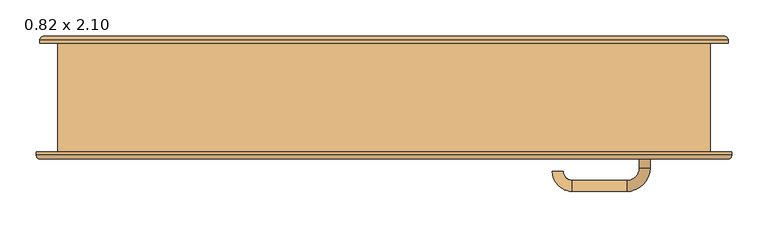
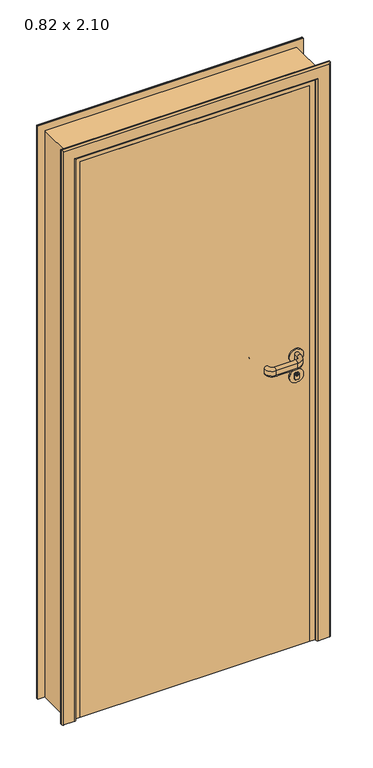
"""IFC4 building model written with IfcOpenShell, lengths in millimetres: door geometry, CC_PORTA ABRIR_1 FOLHA LISA : 0.82 x 2.10."""

from ifc_helpers import new_model, si_unit, point, frame, frame_2d, origin, origin_with_axes, place, context, project, spatial, polyline, circle_curve, ellipse_curve, trimmed, segment, composite_curve, outline, extrude, faceted_brep, source, transform, mapped, element, save
from ifc_brep_helpers import plane_surface, cylinder_surface, revolved_surface, advanced_brep


def door_0_82_x_2_10_6c23dadb(model_context):
    return source(origin(), model_context, "Body", "SolidModel", [
        advanced_brep(
        [(352.5, -40.0, 1091.5062746), (367.5, -40.0, 1091.5062746), (367.5, -40.0, 1108.3826844), (352.5, -40.0, 1108.3826844), (367.5, -18.0, 1091.5062746), (367.5, -18.0, 1108.3826844), (352.5, -18.0, 1108.3826844), (352.5, -18.0, 1091.5062746), (335.0, 14.5, 1108.3826844), (335.0, 14.5, 1091.5062746), (260.0, 14.5, 1091.5062746), (260.0, 14.5, 1108.3826844), (335.0, -0.5, 1091.5062746), (335.0, -0.5, 1108.3826844), (260.0, -0.5, 1108.3826844), (260.0, -0.5, 1091.5062746), (247.5, -13.0, 1091.5062746), (247.5, -13.0, 1108.3826844), (232.5, -13.0, 1108.3826844), (232.5, -13.0, 1091.5062746)],
        [
            (0, 1, circle_curve(frame((360.0, -40.0, 1091.5062746), z_axis=(0.0, -1.0, 0.0), x_axis=(0.0, 0.0, 1.0)), 7.5)),
            (1, 2),
            (2, 3, circle_curve(frame((360.0, -40.0, 1108.3826844), z_axis=(0.0, -1.0, 0.0), x_axis=(0.0, 0.0, 1.0)), 7.5)),
            (3, 0),
            (1, 4),
            (4, 5),
            (5, 2),
            (3, 6),
            (6, 7),
            (7, 0),
            (8, 9),
            (9, 10),
            (10, 11),
            (11, 8),
            (12, 13),
            (13, 14),
            (14, 15),
            (15, 12),
            (7, 4, circle_curve(frame((360.0, -18.0, 1091.5062746), z_axis=(0.0, -1.0, 0.0), x_axis=(0.0, 0.0, 1.0)), 7.5)),
            (5, 6, circle_curve(frame((360.0, -18.0, 1108.3826844), z_axis=(0.0, -1.0, 0.0), x_axis=(0.0, 0.0, 1.0)), 7.5)),
            (9, 12, circle_curve(frame((335.0, 7.0, 1091.5062746), z_axis=(-1.0, 0.0, 0.0), x_axis=(0.0, 0.0, 1.0)), 7.5)),
            (15, 10, circle_curve(frame((260.0, 7.0, 1091.5062746), z_axis=(1.0, 0.0, 0.0), x_axis=(0.0, 0.0, 1.0)), 7.5)),
            (13, 8, circle_curve(frame((335.0, 7.0, 1108.3826844), z_axis=(-1.0, 0.0, 0.0), x_axis=(0.0, 0.0, 1.0)), 7.5)),
            (11, 14, circle_curve(frame((260.0, 7.0, 1108.3826844), z_axis=(1.0, 0.0, 0.0), x_axis=(0.0, 0.0, 1.0)), 7.5)),
            (9, 4, circle_curve(frame((335.0, -18.0, 1091.5062746), z_axis=(0.0, 0.0, -1.0), x_axis=(1.0, 0.0, 0.0)), 32.5)),
            (7, 12, circle_curve(frame((335.0, -18.0, 1091.5062746), z_axis=(0.0, 0.0, 1.0), x_axis=(1.0, 0.0, 0.0)), 17.5)),
            (8, 5, circle_curve(frame((335.0, -18.0, 1108.3826844), z_axis=(0.0, 0.0, -1.0), x_axis=(1.0, 0.0, 0.0)), 32.5)),
            (13, 6, circle_curve(frame((335.0, -18.0, 1108.3826844), z_axis=(0.0, 0.0, -1.0), x_axis=(1.0, 0.0, 0.0)), 17.5)),
            (16, 17),
            (17, 18, circle_curve(frame((240.0, -13.0, 1108.3826844), z_axis=(0.0, -1.0, 0.0), x_axis=(0.0, 0.0, 1.0)), 7.5)),
            (18, 19),
            (19, 16, circle_curve(frame((240.0, -13.0, 1091.5062746), z_axis=(0.0, -1.0, 0.0), x_axis=(0.0, 0.0, 1.0)), 7.5)),
            (19, 10, circle_curve(frame((260.0, -13.0, 1091.5062746), z_axis=(0.0, 0.0, -1.0), x_axis=(0.0, 1.0, 0.0)), 27.5)),
            (15, 16, circle_curve(frame((260.0, -13.0, 1091.5062746), z_axis=(0.0, 0.0, 1.0), x_axis=(0.0, 1.0, 0.0)), 12.5)),
            (18, 11, circle_curve(frame((260.0, -13.0, 1108.3826844), z_axis=(0.0, 0.0, -1.0), x_axis=(0.0, 1.0, 0.0)), 27.5)),
            (17, 14, circle_curve(frame((260.0, -13.0, 1108.3826844), z_axis=(0.0, 0.0, -1.0), x_axis=(0.0, 1.0, 0.0)), 12.5)),
        ],
        [
            plane_surface(frame((360.0, -40.0, 1099.9444795), z_axis=(0.0, -1.0, 0.0), x_axis=(0.0, 0.0, 1.0))),
            plane_surface(frame((367.5, -40.0, 1091.5062746), z_axis=(1.0, 0.0, 0.0), x_axis=(0.0, 1.0, 0.0))),
            plane_surface(frame((352.5, -40.0, 1108.3826844), z_axis=(-1.0, 0.0, 0.0), x_axis=(0.0, 1.0, 0.0))),
            plane_surface(frame((335.0, 14.5, 1091.5062746), z_axis=(0.0, 1.0, 0.0), x_axis=(-1.0, 0.0, 0.0))),
            plane_surface(frame((335.0, -0.5, 1108.3826844), z_axis=(0.0, -1.0, 0.0), x_axis=(-1.0, 0.0, 0.0))),
            cylinder_surface(frame((360.0, -40.0, 1091.5062746), z_axis=(0.0, -1.0, 0.0), x_axis=(0.0, 0.0, 1.0)), 7.5),
            cylinder_surface(frame((360.0, -40.0, 1108.3826844), z_axis=(0.0, -1.0, 0.0), x_axis=(0.0, 0.0, 1.0)), 7.5),
            cylinder_surface(frame((335.0, 7.0, 1091.5062746), z_axis=(1.0, 0.0, 0.0), x_axis=(0.0, 0.0, 1.0)), 7.5),
            cylinder_surface(frame((335.0, 7.0, 1108.3826844), z_axis=(1.0, 0.0, 0.0), x_axis=(0.0, 0.0, 1.0)), 7.5),
            revolved_surface(trimmed(ellipse_curve(frame((360.0, -18.0, 1091.5062746), z_axis=(0.0, -1.0, 0.0), x_axis=(0.0, 0.0, 1.0)), 7.5, 7.5), [point((352.5, -18.0, 1091.5062746))], [point((367.5, -18.0, 1091.5062746))], True, "CARTESIAN"), (335.0, -18.0, 1099.9444795), (0.0, 0.0, 1.0)),
            cylinder_surface(frame((335.0, -18.0, 1099.9444795), z_axis=(0.0, 0.0, 1.0), x_axis=(1.0, 0.0, 0.0)), 32.5),
            revolved_surface(trimmed(ellipse_curve(frame((360.0, -18.0, 1108.3826844), z_axis=(0.0, -1.0, 0.0), x_axis=(0.0, 0.0, 1.0)), 7.5, 7.5), [point((367.5, -18.0, 1108.3826844))], [point((352.5, -18.0, 1108.3826844))], True, "CARTESIAN"), (335.0, -18.0, 1099.9444795), (0.0, 0.0, 1.0)),
            revolved_surface(polyline([(352.5, -18.0, 1108.3826844), (352.5, -18.0, 1091.5062746)]), (335.0, -18.0, 1099.9444795), (0.0, 0.0, 1.0)),
            plane_surface(frame((240.0, -13.0, 1099.9444795), z_axis=(0.0, -1.0, 0.0), x_axis=(0.0, 0.0, 1.0))),
            revolved_surface(trimmed(ellipse_curve(frame((260.0, 7.0, 1091.5062746), z_axis=(1.0, 0.0, 0.0), x_axis=(0.0, 0.0, 1.0)), 7.5, 7.5), [point((260.0, -0.5, 1091.5062746))], [point((260.0, 14.5, 1091.5062746))], True, "CARTESIAN"), (260.0, -13.0, 1099.9444795), (0.0, 0.0, 1.0)),
            cylinder_surface(frame((260.0, -13.0, 1099.9444795), z_axis=(0.0, 0.0, 1.0), x_axis=(0.0, 1.0, 0.0)), 27.5),
            revolved_surface(trimmed(ellipse_curve(frame((260.0, 7.0, 1108.3826844), z_axis=(1.0, 0.0, 0.0), x_axis=(0.0, 0.0, 1.0)), 7.5, 7.5), [point((260.0, 14.5, 1108.3826844))], [point((260.0, -0.5, 1108.3826844))], True, "CARTESIAN"), (260.0, -13.0, 1099.9444795), (0.0, 0.0, 1.0)),
            revolved_surface(polyline([(260.0, -0.5, 1108.3826844), (260.0, -0.5, 1091.5062746)]), (260.0, -13.0, 1099.9444795), (0.0, 0.0, 1.0)),
        ],
        [
            (0, [[1, 2, 3, 4]]),
            (1, [[-2, 5, 6, 7]]),
            (2, [[-4, 8, 9, 10]]),
            (3, [[11, 12, 13, 14]]),
            (4, [[15, 16, 17, 18]]),
            (5, [[-1, -10, 19, -5]]),
            (6, [[-3, -7, 20, -8]]),
            (7, [[21, -18, 22, -12]]),
            (8, [[23, -14, 24, -16]]),
            (9, [[25, -19, 26, -21]]),
            (10, [[27, -6, -25, -11]]),
            (11, [[28, -20, -27, -23]]),
            (12, [[-26, -9, -28, -15]]),
            (13, [[29, 30, 31, 32]]),
            (14, [[33, -22, 34, -32]]),
            (15, [[35, -13, -33, -31]]),
            (16, [[36, -24, -35, -30]]),
            (17, [[-34, -17, -36, -29]]),
        ],
    ),
        extrude(outline(polyline([(361.0, -40.0), (359.0, -40.0), (359.0, -30.9), (361.0, -30.9), (361.0, -40.0)])), frame((0.0, 0.0, 1027.9555433), z_axis=(0.0, 0.0, 1.0), x_axis=(1.0, 0.0, 0.0)), (0.0, 0.0, 1.0), 7.8071257),
        extrude(outline(composite_curve([segment(trimmed(circle_curve(frame_2d((1031.5611613, 360.0)), 5.0), [point((1036.5611613, 360.0))], [point((1026.5611613, 360.0))], False, "CARTESIAN"), True, "CONTINUOUS"), segment(trimmed(circle_curve(frame_2d((1031.5611613, 360.0)), 5.0), [point((1026.5611613, 360.0))], [point((1036.5611613, 360.0))], False, "CARTESIAN"), True, "CONTINUOUS")], self_intersect=False), holes=[polyline([(1035.7626689, 361.0), (1027.9555433, 361.0), (1027.9555433, 359.0), (1035.7626689, 359.0), (1035.7626689, 361.0)])]), frame((0.0, -40.0, 0.0), z_axis=(0.0, 1.0, 0.0), x_axis=(0.0, 0.0, 1.0)), (0.0, 0.0, 1.0), 10.0),
        extrude(outline(composite_curve([segment(polyline([(1033.4817325, 352.5), (1016.4817325, 352.5)]), True, "CONTINUOUS"), segment(trimmed(circle_curve(frame_2d((1016.4817325, 356.5)), 4.0), [point((1016.4817325, 352.5))], [point((1012.4817325, 356.5))], False, "CARTESIAN"), True, "CONTINUOUS"), segment(polyline([(1012.4817325, 356.5), (1012.4817325, 363.5)]), True, "CONTINUOUS"), segment(trimmed(circle_curve(frame_2d((1016.4817325, 363.5)), 4.0), [point((1012.4817325, 363.5))], [point((1016.4817325, 367.5))], False, "CARTESIAN"), True, "CONTINUOUS"), segment(polyline([(1016.4817325, 367.5), (1033.4817325, 367.5)]), True, "CONTINUOUS"), segment(trimmed(circle_curve(frame_2d((1033.4817325, 363.5)), 4.0), [point((1033.4817325, 367.5))], [point((1037.4817325, 363.5))], False, "CARTESIAN"), True, "CONTINUOUS"), segment(polyline([(1037.4817325, 363.5), (1037.4817325, 356.5)]), True, "CONTINUOUS"), segment(trimmed(circle_curve(frame_2d((1033.4817325, 356.5)), 4.0), [point((1037.4817325, 356.5))], [point((1033.4817325, 352.5))], False, "CARTESIAN"), True, "CONTINUOUS")], self_intersect=False)), frame((0.0, -40.0, 0.0), z_axis=(0.0, 1.0, 0.0), x_axis=(0.0, 0.0, 1.0)), (0.0, 0.0, 1.0), 9.0),
        extrude(outline(composite_curve([segment(trimmed(circle_curve(frame_2d((1099.9444795, 360.0)), 25.0), [point((1124.9444795, 360.0))], [point((1074.9444795, 360.0))], False, "CARTESIAN"), True, "CONTINUOUS"), segment(trimmed(circle_curve(frame_2d((1099.9444795, 360.0)), 25.0), [point((1074.9444795, 360.0))], [point((1124.9444795, 360.0))], False, "CARTESIAN"), True, "CONTINUOUS")], self_intersect=False)), frame((0.0, -40.0, 0.0), z_axis=(0.0, 1.0, 0.0), x_axis=(0.0, 0.0, 1.0)), (0.0, 0.0, 1.0), 6.0),
        extrude(outline(composite_curve([segment(trimmed(circle_curve(frame_2d((1024.9444795, 360.0)), 25.0), [point((1049.9444795, 360.0))], [point((999.9444795, 360.0))], False, "CARTESIAN"), True, "CONTINUOUS"), segment(trimmed(circle_curve(frame_2d((1024.9444795, 360.0)), 25.0), [point((999.9444795, 360.0))], [point((1049.9444795, 360.0))], False, "CARTESIAN"), True, "CONTINUOUS")], self_intersect=False), holes=[composite_curve([segment(trimmed(circle_curve(frame_2d((1033.4817325, 363.5)), 4.0), [point((1037.4817325, 363.5))], [point((1033.4817325, 367.5))], True, "CARTESIAN"), True, "CONTINUOUS"), segment(polyline([(1033.4817325, 367.5), (1016.4817325, 367.5)]), True, "CONTINUOUS"), segment(trimmed(circle_curve(frame_2d((1016.4817325, 363.5)), 4.0), [point((1016.4817325, 367.5))], [point((1012.4817325, 363.5))], True, "CARTESIAN"), True, "CONTINUOUS"), segment(polyline([(1012.4817325, 363.5), (1012.4817325, 356.5)]), True, "CONTINUOUS"), segment(trimmed(circle_curve(frame_2d((1016.4817325, 356.5)), 4.0), [point((1012.4817325, 356.5))], [point((1016.4817325, 352.5))], True, "CARTESIAN"), True, "CONTINUOUS"), segment(polyline([(1016.4817325, 352.5), (1033.4817325, 352.5)]), True, "CONTINUOUS"), segment(trimmed(circle_curve(frame_2d((1033.4817325, 356.5)), 4.0), [point((1033.4817325, 352.5))], [point((1037.4817325, 356.5))], True, "CARTESIAN"), True, "CONTINUOUS"), segment(polyline([(1037.4817325, 356.5), (1037.4817325, 363.5)]), True, "CONTINUOUS")], self_intersect=False)]), frame((0.0, -40.0, 0.0), z_axis=(0.0, 1.0, 0.0), x_axis=(0.0, 0.0, 1.0)), (0.0, 0.0, 1.0), 6.0),
        extrude(outline(polyline([(361.0, -84.1), (359.0, -84.1), (359.0, -75.0), (361.0, -75.0), (361.0, -84.1)])), frame((0.0, 0.0, 1027.9555433), z_axis=(0.0, 0.0, 1.0), x_axis=(1.0, 0.0, 0.0)), (0.0, 0.0, 1.0), 7.8071257),
        advanced_brep(
        [(360.0, -85.0, 1036.5611613), (360.0, -85.0, 1026.5611613), (361.0, -85.0, 1035.7626689), (361.0, -85.0, 1027.9555433), (359.0, -85.0, 1027.9555433), (359.0, -85.0, 1035.7626689), (360.0, -75.0, 1049.9444795), (360.0, -75.0, 999.9444795), (360.0, -84.0, 1036.5611613), (360.0, -84.0, 1026.5611613), (361.0, -84.0, 1035.7626689), (361.0, -84.0, 1027.9555433), (359.0, -84.0, 1027.9555433), (359.0, -84.0, 1035.7626689), (352.5, -84.0, 1033.4817325), (352.5, -84.0, 1016.4817325), (356.5, -84.0, 1012.4817325), (363.5, -84.0, 1012.4817325), (367.5, -84.0, 1016.4817325), (367.5, -84.0, 1033.4817325), (363.5, -84.0, 1037.4817325), (356.5, -84.0, 1037.4817325), (352.5, -81.0, 1033.4817325), (352.5, -81.0, 1016.4817325), (356.5, -81.0, 1012.4817325), (363.5, -81.0, 1012.4817325), (367.5, -81.0, 1016.4817325), (367.5, -81.0, 1033.4817325), (363.5, -81.0, 1037.4817325), (356.5, -81.0, 1037.4817325), (360.0, -81.0, 1049.9444795), (360.0, -81.0, 999.9444795)],
        [
            (0, 1, circle_curve(frame((360.0, -85.0, 1031.5611613), z_axis=(0.0, -1.0, 0.0), x_axis=(0.0, 0.0, -1.0)), 5.0)),
            (1, 0, circle_curve(frame((360.0, -85.0, 1031.5611613), z_axis=(0.0, -1.0, 0.0), x_axis=(0.0, 0.0, -1.0)), 5.0)),
            (2, 3),
            (3, 4),
            (4, 5),
            (5, 2),
            (6, 7, circle_curve(frame((360.0, -75.0, 1024.9444795), z_axis=(0.0, 1.0, 0.0), x_axis=(0.0, 0.0, -1.0)), 25.0)),
            (7, 6, circle_curve(frame((360.0, -75.0, 1024.9444795), z_axis=(0.0, 1.0, 0.0), x_axis=(0.0, 0.0, -1.0)), 25.0)),
            (0, 8),
            (8, 9, circle_curve(frame((360.0, -84.0, 1031.5611613), z_axis=(0.0, -1.0, 0.0), x_axis=(0.0, 0.0, -1.0)), 5.0)),
            (9, 1),
            (9, 8, circle_curve(frame((360.0, -84.0, 1031.5611613), z_axis=(0.0, -1.0, 0.0), x_axis=(0.0, 0.0, -1.0)), 5.0)),
            (2, 10),
            (10, 11),
            (11, 3),
            (11, 12),
            (12, 4),
            (12, 13),
            (13, 5),
            (13, 10),
            (14, 15),
            (15, 16, circle_curve(frame((356.5, -84.0, 1016.4817325), z_axis=(0.0, -1.0, 0.0), x_axis=(0.0, 0.0, -1.0)), 4.0)),
            (16, 17),
            (17, 18, circle_curve(frame((363.5, -84.0, 1016.4817325), z_axis=(0.0, -1.0, 0.0), x_axis=(0.0, 0.0, -1.0)), 4.0)),
            (18, 19),
            (19, 20, circle_curve(frame((363.5, -84.0, 1033.4817325), z_axis=(0.0, -1.0, 0.0), x_axis=(0.0, 0.0, -1.0)), 4.0)),
            (20, 21),
            (21, 14, circle_curve(frame((356.5, -84.0, 1033.4817325), z_axis=(0.0, -1.0, 0.0), x_axis=(0.0, 0.0, -1.0)), 4.0)),
            (14, 22),
            (22, 23),
            (23, 15),
            (23, 24, circle_curve(frame((356.5, -81.0, 1016.4817325), z_axis=(0.0, -1.0, 0.0), x_axis=(0.0, 0.0, -1.0)), 4.0)),
            (24, 16),
            (24, 25),
            (25, 17),
            (25, 26, circle_curve(frame((363.5, -81.0, 1016.4817325), z_axis=(0.0, -1.0, 0.0), x_axis=(0.0, 0.0, -1.0)), 4.0)),
            (26, 18),
            (26, 27),
            (27, 19),
            (27, 28, circle_curve(frame((363.5, -81.0, 1033.4817325), z_axis=(0.0, -1.0, 0.0), x_axis=(0.0, 0.0, -1.0)), 4.0)),
            (28, 20),
            (28, 29),
            (29, 21),
            (29, 22, circle_curve(frame((356.5, -81.0, 1033.4817325), z_axis=(0.0, -1.0, 0.0), x_axis=(0.0, 0.0, -1.0)), 4.0)),
            (30, 31, circle_curve(frame((360.0, -81.0, 1024.9444795), z_axis=(0.0, -1.0, 0.0), x_axis=(0.0, 0.0, -1.0)), 25.0)),
            (31, 30, circle_curve(frame((360.0, -81.0, 1024.9444795), z_axis=(0.0, -1.0, 0.0), x_axis=(0.0, 0.0, -1.0)), 25.0)),
            (30, 6),
            (7, 31),
        ],
        [
            plane_surface(frame((360.0, -85.0, 1026.5611613), z_axis=(0.0, -1.0, 0.0), x_axis=(1.0, 0.0, 0.0))),
            plane_surface(frame((360.0, -75.0, 1026.5611613), z_axis=(0.0, 1.0, 0.0), x_axis=(-1.0, 0.0, 0.0))),
            cylinder_surface(frame((360.0, -75.0, 1031.5611613), z_axis=(0.0, -1.0, 0.0), x_axis=(0.0, 0.0, -1.0)), 5.0),
            plane_surface(frame((361.0, -85.0, 1035.7626689), z_axis=(-1.0, 0.0, 0.0), x_axis=(0.0, 1.0, 0.0))),
            plane_surface(frame((361.0, -85.0, 1027.9555433), z_axis=(0.0, 0.0, 1.0), x_axis=(0.0, 1.0, 0.0))),
            plane_surface(frame((359.0, -85.0, 1027.9555433), z_axis=(1.0, 0.0, 0.0), x_axis=(0.0, 1.0, 0.0))),
            plane_surface(frame((359.0, -85.0, 1035.7626689), z_axis=(0.0, 0.0, -1.0), x_axis=(0.0, 1.0, 0.0))),
            plane_surface(frame((352.5, -84.0, 1016.4817325), z_axis=(0.0, -1.0, 0.0), x_axis=(0.0, 0.0, -1.0))),
            plane_surface(frame((352.5, -84.0, 1033.4817325), z_axis=(-1.0, 0.0, 0.0), x_axis=(0.0, 1.0, 0.0))),
            cylinder_surface(frame((356.5, -75.0, 1016.4817325), z_axis=(0.0, -1.0, 0.0), x_axis=(0.0, 0.0, -1.0)), 4.0),
            plane_surface(frame((356.5, -84.0, 1012.4817325), z_axis=(0.0, 0.0, -1.0), x_axis=(0.0, 1.0, 0.0))),
            cylinder_surface(frame((363.5, -75.0, 1016.4817325), z_axis=(0.0, -1.0, 0.0), x_axis=(0.0, 0.0, -1.0)), 4.0),
            plane_surface(frame((367.5, -84.0, 1016.4817325), z_axis=(1.0, 0.0, 0.0), x_axis=(0.0, 1.0, 0.0))),
            cylinder_surface(frame((363.5, -75.0, 1033.4817325), z_axis=(0.0, -1.0, 0.0), x_axis=(0.0, 0.0, -1.0)), 4.0),
            plane_surface(frame((363.5, -84.0, 1037.4817325), z_axis=(0.0, 0.0, 1.0), x_axis=(0.0, 1.0, 0.0))),
            cylinder_surface(frame((356.5, -75.0, 1033.4817325), z_axis=(0.0, -1.0, 0.0), x_axis=(0.0, 0.0, -1.0)), 4.0),
            plane_surface(frame((360.0, -81.0, 1074.9444795), z_axis=(0.0, -1.0, 0.0), x_axis=(1.0, 0.0, 0.0))),
            cylinder_surface(frame((360.0, -75.0, 1024.9444795), z_axis=(0.0, -1.0, 0.0), x_axis=(0.0, 0.0, -1.0)), 25.0),
        ],
        [
            (0, [[1, 2], [3, 4, 5, 6]]),
            (1, [[7, 8]]),
            (2, [[-1, 9, 10, 11]]),
            (2, [[-2, -11, 12, -9]]),
            (3, [[-3, 13, 14, 15]]),
            (4, [[-4, -15, 16, 17]]),
            (5, [[-5, -17, 18, 19]]),
            (6, [[-6, -19, 20, -13]]),
            (7, [[-14, -20, -18, -16]]),
            (7, [[21, 22, 23, 24, 25, 26, 27, 28], [-10, -12]]),
            (8, [[-21, 29, 30, 31]]),
            (9, [[-22, -31, 32, 33]]),
            (10, [[-23, -33, 34, 35]]),
            (11, [[-24, -35, 36, 37]]),
            (12, [[-25, -37, 38, 39]]),
            (13, [[-26, -39, 40, 41]]),
            (14, [[-27, -41, 42, 43]]),
            (15, [[-28, -43, 44, -29]]),
            (16, [[45, 46], [-30, -44, -42, -40, -38, -36, -34, -32]]),
            (17, [[-45, 47, -8, 48]]),
            (17, [[-46, -48, -7, -47]]),
        ],
    ),
        advanced_brep(
        [(360.0, -75.0, 1124.9444795), (360.0, -75.0, 1074.9444795), (360.0, -81.0, 1124.9444795), (360.0, -81.0, 1074.9444795)],
        [
            (0, 1, circle_curve(frame((360.0, -75.0, 1099.9444795), z_axis=(0.0, 1.0, 0.0), x_axis=(0.0, 0.0, -1.0)), 25.0)),
            (1, 0, circle_curve(frame((360.0, -75.0, 1099.9444795), z_axis=(0.0, 1.0, 0.0), x_axis=(0.0, 0.0, -1.0)), 25.0)),
            (2, 3, circle_curve(frame((360.0, -81.0, 1099.9444795), z_axis=(0.0, -1.0, 0.0), x_axis=(0.0, 0.0, -1.0)), 25.0)),
            (3, 2, circle_curve(frame((360.0, -81.0, 1099.9444795), z_axis=(0.0, -1.0, 0.0), x_axis=(0.0, 0.0, -1.0)), 25.0)),
            (2, 0),
            (1, 3),
        ],
        [
            plane_surface(frame((360.0, -75.0, 1026.5611613), z_axis=(0.0, 1.0, 0.0), x_axis=(-1.0, 0.0, 0.0))),
            plane_surface(frame((360.0, -81.0, 1074.9444795), z_axis=(0.0, -1.0, 0.0), x_axis=(1.0, 0.0, 0.0))),
            cylinder_surface(frame((360.0, -75.0, 1099.9444795), z_axis=(0.0, -1.0, 0.0), x_axis=(0.0, 0.0, -1.0)), 25.0),
        ],
        [
            (0, [[1, 2]]),
            (1, [[3, 4]]),
            (2, [[-3, 5, -2, 6]]),
            (2, [[-4, -6, -1, -5]]),
        ],
    ),
        advanced_brep(
        [(352.5, -75.0, 1108.4382049), (367.5, -75.0, 1108.4382049), (367.5, -75.0, 1091.5617951), (352.5, -75.0, 1091.5617951), (367.5, -97.0, 1108.4382049), (367.5, -97.0, 1091.5617951), (352.5, -97.0, 1091.5617951), (352.5, -97.0, 1108.4382049), (335.0, -129.5, 1091.5617951), (335.0, -129.5, 1108.4382049), (260.0, -129.5, 1108.4382049), (260.0, -129.5, 1091.5617951), (335.0, -114.5, 1108.4382049), (335.0, -114.5, 1091.5617951), (260.0, -114.5, 1091.5617951), (260.0, -114.5, 1108.4382049), (247.5, -102.0, 1108.4382049), (247.5, -102.0, 1091.5617951), (232.5, -102.0, 1091.5617951), (232.5, -102.0, 1108.4382049)],
        [
            (0, 1, circle_curve(frame((360.0, -75.0, 1108.4382049), z_axis=(0.0, 1.0, 0.0), x_axis=(-1.0, 0.0, 0.0)), 7.5)),
            (1, 2),
            (2, 3, circle_curve(frame((360.0, -75.0, 1091.5617951), z_axis=(0.0, 1.0, 0.0), x_axis=(-1.0, 0.0, 0.0)), 7.5)),
            (3, 0),
            (1, 4),
            (4, 5),
            (5, 2),
            (3, 6),
            (6, 7),
            (7, 0),
            (8, 9),
            (9, 10),
            (10, 11),
            (11, 8),
            (12, 13),
            (13, 14),
            (14, 15),
            (15, 12),
            (7, 4, circle_curve(frame((360.0, -97.0, 1108.4382049), z_axis=(0.0, 1.0, 0.0), x_axis=(-1.0, 0.0, 0.0)), 7.5)),
            (5, 6, circle_curve(frame((360.0, -97.0, 1091.5617951), z_axis=(0.0, 1.0, 0.0), x_axis=(-1.0, 0.0, 0.0)), 7.5)),
            (9, 12, circle_curve(frame((335.0, -122.0, 1108.4382049), z_axis=(-1.0, 0.0, 0.0), x_axis=(0.0, 1.0, 0.0)), 7.5)),
            (15, 10, circle_curve(frame((260.0, -122.0, 1108.4382049), z_axis=(1.0, 0.0, 0.0), x_axis=(0.0, 1.0, 0.0)), 7.5)),
            (13, 8, circle_curve(frame((335.0, -122.0, 1091.5617951), z_axis=(-1.0, 0.0, 0.0), x_axis=(0.0, 1.0, 0.0)), 7.5)),
            (11, 14, circle_curve(frame((260.0, -122.0, 1091.5617951), z_axis=(1.0, 0.0, 0.0), x_axis=(0.0, 1.0, 0.0)), 7.5)),
            (9, 4, circle_curve(frame((335.0, -97.0, 1108.4382049), z_axis=(0.0, 0.0, 1.0), x_axis=(1.0, 0.0, 0.0)), 32.5)),
            (7, 12, circle_curve(frame((335.0, -97.0, 1108.4382049), z_axis=(0.0, 0.0, -1.0), x_axis=(1.0, 0.0, 0.0)), 17.5)),
            (8, 5, circle_curve(frame((335.0, -97.0, 1091.5617951), z_axis=(0.0, 0.0, 1.0), x_axis=(1.0, 0.0, 0.0)), 32.5)),
            (13, 6, circle_curve(frame((335.0, -97.0, 1091.5617951), z_axis=(0.0, 0.0, 1.0), x_axis=(1.0, 0.0, 0.0)), 17.5)),
            (16, 17),
            (17, 18, circle_curve(frame((240.0, -102.0, 1091.5617951), z_axis=(0.0, 1.0, 0.0), x_axis=(1.0, 0.0, 0.0)), 7.5)),
            (18, 19),
            (19, 16, circle_curve(frame((240.0, -102.0, 1108.4382049), z_axis=(0.0, 1.0, 0.0), x_axis=(1.0, 0.0, 0.0)), 7.5)),
            (19, 10, circle_curve(frame((260.0, -102.0, 1108.4382049), z_axis=(0.0, 0.0, 1.0), x_axis=(0.0, -1.0, 0.0)), 27.5)),
            (15, 16, circle_curve(frame((260.0, -102.0, 1108.4382049), z_axis=(0.0, 0.0, -1.0), x_axis=(0.0, -1.0, 0.0)), 12.5)),
            (18, 11, circle_curve(frame((260.0, -102.0, 1091.5617951), z_axis=(0.0, 0.0, 1.0), x_axis=(0.0, -1.0, 0.0)), 27.5)),
            (17, 14, circle_curve(frame((260.0, -102.0, 1091.5617951), z_axis=(0.0, 0.0, 1.0), x_axis=(0.0, -1.0, 0.0)), 12.5)),
        ],
        [
            plane_surface(frame((360.0, -75.0, 1100.0), z_axis=(0.0, 1.0, 0.0), x_axis=(0.0, 0.0, -1.0))),
            plane_surface(frame((367.5, -75.0, 1108.4382049), z_axis=(1.0, 0.0, 0.0), x_axis=(0.0, -1.0, 0.0))),
            plane_surface(frame((352.5, -75.0, 1091.5617951), z_axis=(-1.0, 0.0, 0.0), x_axis=(0.0, -1.0, 0.0))),
            plane_surface(frame((335.0, -129.5, 1108.4382049), z_axis=(0.0, -1.0, 0.0), x_axis=(-1.0, 0.0, 0.0))),
            plane_surface(frame((335.0, -114.5, 1091.5617951), z_axis=(0.0, 1.0, 0.0), x_axis=(-1.0, 0.0, 0.0))),
            cylinder_surface(frame((360.0, -75.0, 1108.4382049), z_axis=(0.0, 1.0, 0.0), x_axis=(-1.0, 0.0, 0.0)), 7.5),
            cylinder_surface(frame((360.0, -75.0, 1091.5617951), z_axis=(0.0, 1.0, 0.0), x_axis=(-1.0, 0.0, 0.0)), 7.5),
            cylinder_surface(frame((335.0, -122.0, 1108.4382049), z_axis=(1.0, 0.0, 0.0), x_axis=(0.0, 1.0, 0.0)), 7.5),
            cylinder_surface(frame((335.0, -122.0, 1091.5617951), z_axis=(1.0, 0.0, 0.0), x_axis=(0.0, 1.0, 0.0)), 7.5),
            revolved_surface(trimmed(ellipse_curve(frame((360.0, -97.0, 1108.4382049), z_axis=(0.0, 1.0, 0.0), x_axis=(-1.0, 0.0, 0.0)), 7.5, 7.5), [point((352.5, -97.0, 1108.4382049))], [point((367.5, -97.0, 1108.4382049))], True, "CARTESIAN"), (335.0, -97.0, 1100.0), (0.0, 0.0, -1.0)),
            cylinder_surface(frame((335.0, -97.0, 1100.0), z_axis=(0.0, 0.0, -1.0), x_axis=(1.0, 0.0, 0.0)), 32.5),
            revolved_surface(trimmed(ellipse_curve(frame((360.0, -97.0, 1091.5617951), z_axis=(0.0, 1.0, 0.0), x_axis=(-1.0, 0.0, 0.0)), 7.5, 7.5), [point((367.5, -97.0, 1091.5617951))], [point((352.5, -97.0, 1091.5617951))], True, "CARTESIAN"), (335.0, -97.0, 1100.0), (0.0, 0.0, -1.0)),
            revolved_surface(polyline([(352.5, -97.0, 1091.5617951), (352.5, -97.0, 1108.4382049)]), (335.0, -97.0, 1100.0), (0.0, 0.0, -1.0)),
            plane_surface(frame((240.0, -102.0, 1100.0), z_axis=(0.0, 1.0, 0.0), x_axis=(0.0, 0.0, -1.0))),
            revolved_surface(trimmed(ellipse_curve(frame((260.0, -122.0, 1108.4382049), z_axis=(1.0, 0.0, 0.0), x_axis=(0.0, 1.0, 0.0)), 7.5, 7.5), [point((260.0, -114.5, 1108.4382049))], [point((260.0, -129.5, 1108.4382049))], True, "CARTESIAN"), (260.0, -102.0, 1100.0), (0.0, 0.0, -1.0)),
            cylinder_surface(frame((260.0, -102.0, 1100.0), z_axis=(0.0, 0.0, -1.0), x_axis=(0.0, -1.0, 0.0)), 27.5),
            revolved_surface(trimmed(ellipse_curve(frame((260.0, -122.0, 1091.5617951), z_axis=(1.0, 0.0, 0.0), x_axis=(0.0, 1.0, 0.0)), 7.5, 7.5), [point((260.0, -129.5, 1091.5617951))], [point((260.0, -114.5, 1091.5617951))], True, "CARTESIAN"), (260.0, -102.0, 1100.0), (0.0, 0.0, -1.0)),
            revolved_surface(polyline([(260.0, -114.5, 1091.5617951), (260.0, -114.5, 1108.4382049)]), (260.0, -102.0, 1100.0), (0.0, 0.0, -1.0)),
        ],
        [
            (0, [[1, 2, 3, 4]]),
            (1, [[-2, 5, 6, 7]]),
            (2, [[-4, 8, 9, 10]]),
            (3, [[11, 12, 13, 14]]),
            (4, [[15, 16, 17, 18]]),
            (5, [[-1, -10, 19, -5]]),
            (6, [[-3, -7, 20, -8]]),
            (7, [[21, -18, 22, -12]]),
            (8, [[23, -14, 24, -16]]),
            (9, [[25, -19, 26, -21]]),
            (10, [[27, -6, -25, -11]]),
            (11, [[28, -20, -27, -23]]),
            (12, [[-26, -9, -28, -15]]),
            (13, [[29, 30, 31, 32]]),
            (14, [[33, -22, 34, -32]]),
            (15, [[35, -13, -33, -31]]),
            (16, [[36, -24, -35, -30]]),
            (17, [[-34, -17, -36, -29]]),
        ],
    ),
        extrude(outline(polyline([(410.0, -75.0), (-410.0, -75.0), (-410.0, -40.0), (410.0, -40.0), (410.0, -75.0)])), origin_with_axes(), (0.0, 0.0, 1.0), 2100.0),
        advanced_brep(
        [(-430.5, 85.0, 0.0), (-425.0, 79.5, 0.0), (-425.0, 75.0, 0.0), (-475.0, 75.0, 0.0), (-475.0, 79.500573, 0.0), (-469.500573, 85.0, 0.0), (-430.5, 85.0, 2120.5), (-425.0, 79.5, 2115.0), (-425.0, 75.0, 2115.0), (425.0, 75.0, 2115.0), (425.0, 75.0, 0.0), (475.0, 75.0, 0.0), (475.0, 75.0, 2165.0), (-475.0, 75.0, 2165.0), (-475.0, 79.500573, 2165.0), (-469.500573, 85.0, 2159.500573), (469.500573, 85.0, 2159.500573), (469.500573, 85.0, 0.0), (430.5, 85.0, 0.0), (430.5, 85.0, 2120.5), (425.0, 79.5, 2115.0), (425.0, 79.5, 0.0), (475.0, 79.500573, 0.0), (475.0, 79.500573, 2165.0)],
        [
            (0, 1, circle_curve(frame((-430.5, 79.5, 0.0), z_axis=(0.0, 0.0, -1.0), x_axis=(0.0, 1.0, 0.0)), 5.5)),
            (1, 2),
            (2, 3),
            (3, 4),
            (4, 5, circle_curve(frame((-469.500573, 79.500573, 0.0), z_axis=(0.0, 0.0, -1.0), x_axis=(0.0, 1.0, 0.0)), 5.499427)),
            (5, 0),
            (0, 6),
            (6, 7, ellipse_curve(frame((-430.5, 79.5, 2120.5), z_axis=(-0.7071067811865475, 0.0, -0.7071067811865476), x_axis=(0.7071067811865476, 0.0, -0.7071067811865474)), 7.7781746, 5.5)),
            (7, 1),
            (7, 8),
            (8, 2),
            (8, 9),
            (9, 10),
            (10, 11),
            (11, 12),
            (12, 13),
            (13, 3),
            (13, 14),
            (14, 4),
            (14, 15, ellipse_curve(frame((-469.500573, 79.500573, 2159.500573), z_axis=(-0.7071067811865475, 0.0, -0.7071067811865476), x_axis=(0.7071067811865476, 0.0, -0.7071067811865474)), 7.7773642, 5.499427)),
            (15, 5),
            (15, 16),
            (16, 17),
            (17, 18),
            (18, 19),
            (19, 6),
            (9, 20),
            (20, 21),
            (21, 10),
            (17, 22, circle_curve(frame((469.500573, 79.500573, 0.0), z_axis=(0.0, 0.0, -1.0), x_axis=(0.0, 1.0, 0.0)), 5.499427)),
            (22, 11),
            (21, 18, circle_curve(frame((430.5, 79.5, 0.0), z_axis=(0.0, 0.0, -1.0), x_axis=(0.0, 1.0, 0.0)), 5.5)),
            (23, 12),
            (22, 23),
            (16, 23, ellipse_curve(frame((469.500573, 79.500573, 2159.500573), z_axis=(0.7071067811865475, 0.0, -0.7071067811865475), x_axis=(0.7071067811865474, 0.0, 0.7071067811865477)), 7.7773642, 5.499427)),
            (20, 19, ellipse_curve(frame((430.5, 79.5, 2120.5), z_axis=(0.7071067811865475, 0.0, -0.7071067811865475), x_axis=(0.7071067811865474, 0.0, 0.7071067811865477)), 7.7781746, 5.5)),
            (20, 7),
            (23, 14),
        ],
        [
            plane_surface(frame((-450.0, 75.0, 0.0), z_axis=(0.0, 0.0, -1.0), x_axis=(-1.0, 0.0, 0.0))),
            cylinder_surface(frame((-430.5, 79.5, 0.0), z_axis=(0.0, 0.0, -1.0), x_axis=(0.0, 1.0, 0.0)), 5.5),
            plane_surface(frame((-425.0, 79.5, 0.0), z_axis=(1.0, 0.0, 0.0), x_axis=(0.0, 0.0, 1.0))),
            plane_surface(frame((-425.0, 75.0, 0.0), z_axis=(0.0, -1.0, 0.0), x_axis=(0.0, 0.0, 1.0))),
            plane_surface(frame((-475.0, 75.0, 0.0), z_axis=(-1.0, 0.0, 0.0), x_axis=(0.0, 0.0, 1.0))),
            cylinder_surface(frame((-469.500573, 79.500573, 0.0), z_axis=(0.0, 0.0, -1.0), x_axis=(0.0, 1.0, 0.0)), 5.499427),
            plane_surface(frame((-469.500573, 85.0, 0.0), z_axis=(0.0, 1.0, 0.0), x_axis=(0.0, 0.0, 1.0))),
            plane_surface(frame((425.0, 79.5, 2115.0), z_axis=(-1.0, 0.0, 0.0), x_axis=(0.0, 0.0, -1.0))),
            plane_surface(frame((450.0, 75.0, 0.0), z_axis=(0.0, 0.0, -1.0), x_axis=(1.0, 0.0, 0.0))),
            plane_surface(frame((475.0, 75.0, 2165.0), z_axis=(1.0, 0.0, 0.0), x_axis=(0.0, 0.0, -1.0))),
            cylinder_surface(frame((469.500573, 79.500573, 2140.0), z_axis=(0.0, 0.0, 1.0), x_axis=(0.0, 1.0, 0.0)), 5.499427),
            cylinder_surface(frame((430.5, 79.5, 2140.0), z_axis=(0.0, 0.0, 1.0), x_axis=(0.0, 1.0, 0.0)), 5.5),
            cylinder_surface(frame((-450.0, 79.5, 2120.5), z_axis=(-1.0, 0.0, 0.0), x_axis=(0.0, 1.0, 0.0)), 5.5),
            plane_surface(frame((-425.0, 79.5, 2115.0), z_axis=(0.0, 0.0, -1.0), x_axis=(1.0, 0.0, 0.0))),
            plane_surface(frame((-475.0, 75.0, 2165.0), z_axis=(0.0, 0.0, 1.0), x_axis=(1.0, 0.0, 0.0))),
            cylinder_surface(frame((-450.0, 79.500573, 2159.500573), z_axis=(-1.0, 0.0, 0.0), x_axis=(0.0, 1.0, 0.0)), 5.499427),
        ],
        [
            (0, [[1, 2, 3, 4, 5, 6]]),
            (1, [[-1, 7, 8, 9]]),
            (2, [[-2, -9, 10, 11]]),
            (3, [[-3, -11, 12, 13, 14, 15, 16, 17]]),
            (4, [[-4, -17, 18, 19]]),
            (5, [[-5, -19, 20, 21]]),
            (6, [[-6, -21, 22, 23, 24, 25, 26, -7]]),
            (7, [[27, 28, 29, -13]]),
            (8, [[-24, 30, 31, -14, -29, 32]]),
            (9, [[33, -15, -31, 34]]),
            (10, [[35, -34, -30, -23]]),
            (11, [[36, -25, -32, -28]]),
            (12, [[-8, -26, -36, 37]]),
            (13, [[-10, -37, -27, -12]]),
            (14, [[-18, -16, -33, 38]]),
            (15, [[-20, -38, -35, -22]]),
        ],
    ),
        advanced_brep(
        [(-430.0, -75.0, 0.0), (-430.0, -79.5, 0.0), (-435.5, -85.0, 0.0), (-474.5, -85.0, 0.0), (-480.0, -79.5, 0.0), (-480.0, -75.0, 0.0), (-430.0, -75.0, 2120.0), (-430.0, -79.5, 2120.0), (-435.5, -85.0, 2125.5), (435.5, -85.0, 2125.5), (435.5, -85.0, 0.0), (474.5, -85.0, 0.0), (474.5, -85.0, 2164.5), (-474.5, -85.0, 2164.5), (-480.0, -79.5, 2170.0), (-480.0, -75.0, 2170.0), (480.0, -75.0, 2170.0), (480.0, -75.0, 0.0), (430.0, -75.0, 0.0), (430.0, -75.0, 2120.0), (430.0, -79.5, 2120.0), (430.0, -79.5, 0.0), (480.0, -79.5, 0.0), (480.0, -79.5, 2170.0)],
        [
            (0, 1),
            (1, 2, circle_curve(frame((-435.5, -79.5, 0.0), z_axis=(0.0, 0.0, -1.0), x_axis=(0.0, 1.0, 0.0)), 5.5)),
            (2, 3),
            (3, 4, circle_curve(frame((-474.5, -79.5, 0.0), z_axis=(0.0, 0.0, -1.0), x_axis=(0.0, 1.0, 0.0)), 5.5)),
            (4, 5),
            (5, 0),
            (0, 6),
            (6, 7),
            (7, 1),
            (7, 8, ellipse_curve(frame((-435.5, -79.5, 2125.5), z_axis=(-0.7071067811865475, 0.0, -0.7071067811865476), x_axis=(0.7071067811865476, 0.0, -0.7071067811865474)), 7.7781746, 5.5)),
            (8, 2),
            (8, 9),
            (9, 10),
            (10, 11),
            (11, 12),
            (12, 13),
            (13, 3),
            (13, 14, ellipse_curve(frame((-474.5, -79.5, 2164.5), z_axis=(-0.7071067811865475, 0.0, -0.7071067811865476), x_axis=(0.7071067811865476, 0.0, -0.7071067811865474)), 7.7781746, 5.5)),
            (14, 4),
            (14, 15),
            (15, 5),
            (15, 16),
            (16, 17),
            (17, 18),
            (18, 19),
            (19, 6),
            (9, 20, ellipse_curve(frame((435.5, -79.5, 2125.5), z_axis=(0.7071067811865475, 0.0, -0.7071067811865475), x_axis=(0.7071067811865474, 0.0, 0.7071067811865477)), 7.7781746, 5.5)),
            (20, 21),
            (21, 10, circle_curve(frame((435.5, -79.5, 0.0), z_axis=(0.0, 0.0, 1.0), x_axis=(0.0, 1.0, 0.0)), 5.5)),
            (17, 22),
            (22, 11, circle_curve(frame((474.5, -79.5, 0.0), z_axis=(0.0, 0.0, -1.0), x_axis=(0.0, 1.0, 0.0)), 5.5)),
            (21, 18),
            (23, 12, ellipse_curve(frame((474.5, -79.5, 2164.5), z_axis=(0.7071067811865475, 0.0, -0.7071067811865475), x_axis=(0.7071067811865474, 0.0, 0.7071067811865477)), 7.7781746, 5.5)),
            (22, 23),
            (16, 23),
            (20, 19),
            (20, 7),
            (23, 14),
        ],
        [
            plane_surface(frame((-450.0, -75.0, 0.0), z_axis=(0.0, 0.0, -1.0), x_axis=(-1.0, 0.0, 0.0))),
            plane_surface(frame((-430.0, -75.0, 0.0), z_axis=(1.0, 0.0, 0.0), x_axis=(0.0, 0.0, 1.0))),
            cylinder_surface(frame((-435.5, -79.5, 0.0), z_axis=(0.0, 0.0, -1.0), x_axis=(0.0, 1.0, 0.0)), 5.5),
            plane_surface(frame((-435.5, -85.0, 0.0), z_axis=(0.0, -1.0, 0.0), x_axis=(0.0, 0.0, 1.0))),
            cylinder_surface(frame((-474.5, -79.5, 0.0), z_axis=(0.0, 0.0, -1.0), x_axis=(0.0, 1.0, 0.0)), 5.5),
            plane_surface(frame((-480.0, -79.5, 0.0), z_axis=(-1.0, 0.0, 0.0), x_axis=(0.0, 0.0, 1.0))),
            plane_surface(frame((-480.0, -75.0, 0.0), z_axis=(0.0, 1.0, 0.0), x_axis=(0.0, 0.0, 1.0))),
            cylinder_surface(frame((435.5, -79.5, 2140.0), z_axis=(0.0, 0.0, 1.0), x_axis=(0.0, 1.0, 0.0)), 5.5),
            plane_surface(frame((450.0, -75.0, 0.0), z_axis=(0.0, 0.0, -1.0), x_axis=(1.0, 0.0, 0.0))),
            cylinder_surface(frame((474.5, -79.5, 2140.0), z_axis=(0.0, 0.0, 1.0), x_axis=(0.0, 1.0, 0.0)), 5.5),
            plane_surface(frame((480.0, -79.5, 2170.0), z_axis=(1.0, 0.0, 0.0), x_axis=(0.0, 0.0, -1.0))),
            plane_surface(frame((430.0, -75.0, 2120.0), z_axis=(-1.0, 0.0, 0.0), x_axis=(0.0, 0.0, -1.0))),
            plane_surface(frame((-430.0, -75.0, 2120.0), z_axis=(0.0, 0.0, -1.0), x_axis=(1.0, 0.0, 0.0))),
            cylinder_surface(frame((-450.0, -79.5, 2125.5), z_axis=(-1.0, 0.0, 0.0), x_axis=(0.0, 1.0, 0.0)), 5.5),
            cylinder_surface(frame((-450.0, -79.5, 2164.5), z_axis=(-1.0, 0.0, 0.0), x_axis=(0.0, 1.0, 0.0)), 5.5),
            plane_surface(frame((-480.0, -79.5, 2170.0), z_axis=(0.0, 0.0, 1.0), x_axis=(1.0, 0.0, 0.0))),
        ],
        [
            (0, [[1, 2, 3, 4, 5, 6]]),
            (1, [[-1, 7, 8, 9]]),
            (2, [[-2, -9, 10, 11]]),
            (3, [[-3, -11, 12, 13, 14, 15, 16, 17]]),
            (4, [[-4, -17, 18, 19]]),
            (5, [[-5, -19, 20, 21]]),
            (6, [[-6, -21, 22, 23, 24, 25, 26, -7]]),
            (7, [[27, 28, 29, -13]]),
            (8, [[-24, 30, 31, -14, -29, 32]]),
            (9, [[33, -15, -31, 34]]),
            (10, [[35, -34, -30, -23]]),
            (11, [[36, -25, -32, -28]]),
            (12, [[-8, -26, -36, 37]]),
            (13, [[-10, -37, -27, -12]]),
            (14, [[-18, -16, -33, 38]]),
            (15, [[-20, -38, -35, -22]]),
        ],
    ),
        faceted_brep([(-410.0, -40.0, 0.0), (-410.0, -75.0, 0.0), (-450.0, -75.0, 0.0), (-450.0, 75.0, 0.0), (-400.0, 75.0, 0.0), (-400.0, -40.0, 0.0), (-410.0, -40.0, 2100.0), (-410.0, -75.0, 2100.0), (410.0, -75.0, 2100.0), (410.0, -75.0, 0.0), (450.0, -75.0, 0.0), (450.0, -75.0, 2140.0), (-450.0, -75.0, 2140.0), (-450.0, 75.0, 2140.0), (450.0, 75.0, 2140.0), (450.0, 75.0, 0.0), (400.0, 75.0, 0.0), (400.0, 75.0, 2090.0), (-400.0, 75.0, 2090.0), (-400.0, -40.0, 2090.0), (400.0, -40.0, 2090.0), (400.0, -40.0, 0.0), (410.0, -40.0, 0.0), (410.0, -40.0, 2100.0)], [[[0, 1, 2, 3, 4, 5]], [[1, 0, 6, 7]], [[2, 1, 7, 8, 9, 10, 11, 12]], [[3, 2, 12, 13]], [[4, 3, 13, 14, 15, 16, 17, 18]], [[5, 4, 18, 19]], [[0, 5, 19, 20, 21, 22, 23, 6]], [[8, 23, 22, 9]], [[22, 21, 16, 15, 10, 9]], [[14, 11, 10, 15]], [[20, 17, 16, 21]], [[7, 6, 23, 8]], [[13, 12, 11, 14]], [[19, 18, 17, 20]]]),
    ])


if __name__ == "__main__":
    model = new_model("IFC4")
    model_context = context("Model", 3, world=origin())
    ifc_project = project(units=[si_unit("LENGTHUNIT", "METRE", prefix="MILLI")], contexts=[model_context])
    site = spatial("IfcSite", under=ifc_project)
    building = spatial("IfcBuilding", under=site)
    placement = place(None, origin())
    door_0_82_x_2_10_shape = door_0_82_x_2_10_6c23dadb(model_context)
    element("IfcDoor", 1, ObjectType="CC_PORTA ABRIR_1 FOLHA LISA : 0.82 x 2.10", at=placement, inside=building, context=model_context, shape_type="MappedRepresentation", body=[
        mapped(door_0_82_x_2_10_shape, transform((0.0, 0.0, 0.0), x_axis=(1.0, 0.0, 0.0), y_axis=(0.0, 1.0, 0.0), z_axis=(0.0, 0.0, 1.0))),
    ])
    save(model, "model.ifc")

# Revit data of these elements
# Type "CC_PORTA ABRIR_1 FOLHA LISA : 0.82 x 2.10"
#   Type Mark = "P2"
#   Site = "www.construir.arq.br"
#   Empresa = "Cursos Construir"
#   Description = "PORTA ABRIR 1 FOLHA LISA"
#   Criado Por = "Roberto Netto"
#   Analytic Construction = "<Nenhum>"
#   Atualizado por = "Rudemberg Eloi"
#   Rough Width = 0.90 m
#   Interna [instance default] = 0.00 m
#   Largura Guarnição Interna [instance default] = 0.05 m
#   Largura Guarnição Externa [instance default] = 0.05 m
#   Largura Folha [instance default] = 0.82 m
#   Externa [instance default] = 0.00 m
#   Extensão Lateral Esquerda [instance default] = 0.03 m
#   Extensão Lateral Direita [instance default] = 0.03 m
#   Extensão Frontal [instance default] = 0.03 m
#   Espessura Soleira [instance default] = 0.02 m
#   Espessura Guarnição Interna [instance default] = 0.01 m
#   Espessura Guarnição Externa [instance default] = 0.01 m
#   Espessura Folha [instance default] = 0.035 m
#   Espessura Batente [instance default] = 0.05 m
#   Eixo Rotação Folha [instance default] = 0.04 m
#   Deslocamento Maçaneta [instance default] = 0.05 m
#   Deslocamento Fechadura [instance default] = 0.05 m
#   Desloc (Interno) [instance default] = 0.02 m
#   Desloc (Externo) [instance default] = 0.025 m
#   Rough Height = 2.14 m
#   Altura Maçaneta [instance default] = 1.10 m
#   Altura Folha [instance default] = 2.10 m
#   Altura Fechadura [instance default] = 1.00 m
#   Height = 2.14 m
#   Width = 0.90 m
#   ----SOLEIRA---- [instance default] = 0.00 m
#   ----MAÇANETA/FECHADURA---- [instance default] = 0.00 m
#   ----GUARNIÇÃO---- [instance default] = 0.00 m
#   ----FOLHA---- [instance default] = 0.00 m
#   ----EXTENSÃO---- [instance default] = 0.00 m
#   ----BATENTE---- [instance default] = 0.00 m
#   Soleira Sem Extensão [instance default] = yes
#   Soleira Com Extensão [instance default] = no
#   Soleira [instance default] = yes
#   Maçaneta / Puxador [instance default] = yes
#   Guarnição Interna [instance default] = yes
#   Guarnição Externa [instance default] = yes
#   Fechadura Separada [instance default] = no
#   Bit [instance default] = no
#   Porcent. Exibição Batente Interno [instance default] = 50
#   Porcent. Exibição Batente Externo [instance default] = 50
#   Material Bit/Soleira = .GRANITO BRANCO ITAÚNAS
#   Material Espelho/Fixação = .AÇO INOXIDÁVEL ESCOVADO
#   Material Maçaneta/Puxador = .AÇO INOXIDÁVEL ESCOVADO
#   Material Guarnição Interna = .MADEIRA COM PINTURA ESMALTE BRANCO ACETINADO
#   Material Guarnição Externa = .MADEIRA COM PINTURA ESMALTE BRANCO ACETINADO
#   Material Folha = .MADEIRA COM PINTURA ESMALTE BRANCO ACETINADO
#   Material Fechadura = .AÇO INOXIDÁVEL ESCOVADO
#   Material Batente = .MADEIRA COM PINTURA ESMALTE BRANCO ACETINADO
#   Família Maçaneta [instance default] = element 613477
#   Function = (empty or 0)
#   Wall Closure = (empty or 0)
# Element 1 (IfcDoor, "CC_PORTA ABRIR_1 FOLHA LISA : 0.82 x 2.10")
#   Materials on its faces: ".AÇO INOXIDÁVEL ESCOVADO", ".MADEIRA COM PINTURA ESMALTE BRANCO ACETINADO"
# Materials
#   ".GRANITO BRANCO ITAÚNAS": class ".CC_PEDRA REVEST.", colour RGB 202 195 174, transparency 0, Description = "Granito branco Itaúnas", Uso = "Pedra", Cost = 0
#   ".AÇO INOXIDÁVEL ESCOVADO": class "Metal", colour RGB 189 187 185, transparency 0, Description = "Stainless Steel 18/8, brushed finish", Cost = 0
#   ".MADEIRA COM PINTURA ESMALTE BRANCO ACETINADO": class ".CC_MADEIRAS", colour RGB 240 240 240, transparency 0, Description = "Madeira com pintura esmalte branco acetinado.", Cost = 0
